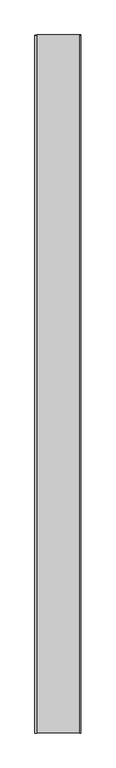
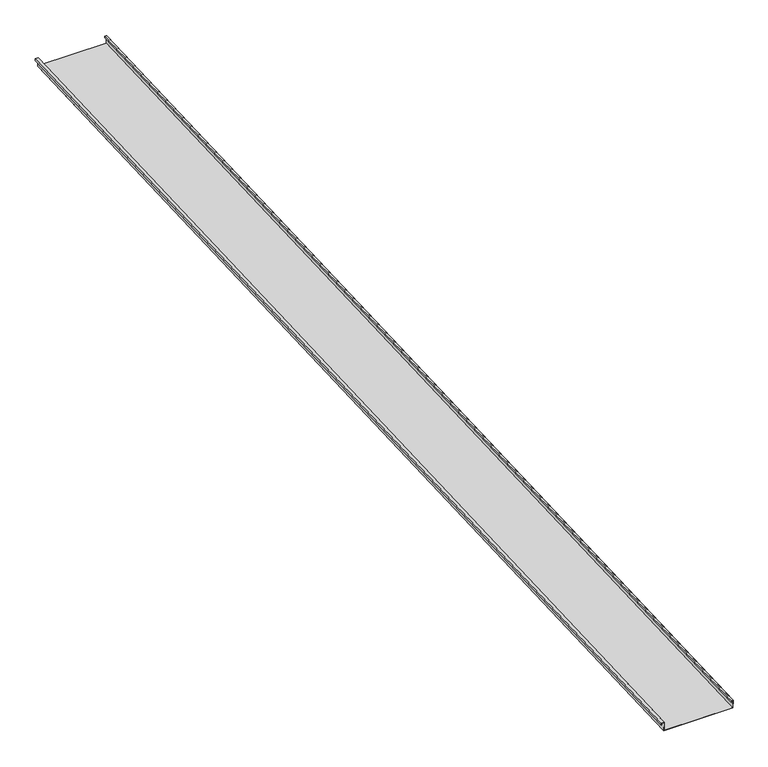
"""IFC4 building model written with IfcOpenShell, lengths in millimetres: proxy geometry, Generic Models 2:Generic Models 2:310765:Generic Models 2:310765 : Generic Models 2:Generic Models 2:310765:124 : Generic Models 2:Generic Models 2:310765:Generic Models 2:310765 : Generic Models 2:Generic Models 2:310765:300385."""

from ifc_helpers import new_model, si_unit, frame, origin, place, context, project, spatial, polyline, outline, extrude, source, transform, mapped, element, save


def generic_models_ac668154(model_context):
    return source(origin(), model_context, "Body", "SweptSolid", [
        extrude(outline(polyline([(1.5875, 0.0), (1.5875, 50.8), (407.9875, 50.8), (407.9875, 1.5875), (396.875, 1.5875), (396.875, 11.1125), (398.4625, 11.1125), (398.4625, 3.175), (406.4, 3.175), (406.4, 49.2125), (3.175, 49.2125), (3.175, -1.5874999), (-14.2875, -1.5874999), (-14.2875, 9.525), (-12.7, 9.525), (-12.7, 0.0), (1.5875, 0.0)])), frame((662984.0429738, -581354.4345603, 3902.6697972), z_axis=(0.0, 0.9991330730923568, 0.041630544712067834), x_axis=(1.0, 0.0, 0.0)), (0.0, 0.0, 1.0), 6400.8),
    ])


if __name__ == "__main__":
    model = new_model("IFC4")
    model_context = context("Model", 3, world=origin())
    ifc_project = project(units=[si_unit("LENGTHUNIT", "METRE", prefix="MILLI")], contexts=[model_context])
    site = spatial("IfcSite", under=ifc_project)
    building = spatial("IfcBuilding", under=site)
    placement = place(None, origin())
    generic_models_shape = generic_models_ac668154(model_context)
    element("IfcBuildingElementProxy", 1, Name="Generic Models 2:Generic Models 2:310765:Generic Models 2:310765 : Generic Models 2:Generic Models 2:310765:124 : Generic Models 2:Generic Models 2:310765:Generic Models 2:310765 : Generic Models 2:Generic Models 2:310765:300385", ObjectType="Generic Models 2:Generic Models 2:310765:Generic Models 2:310765 : Generic Models 2:Generic Models 2:310765:124 : Generic Models 2:Generic Models 2:310765:Generic Models 2:310765 : Generic Models 2:Generic Models 2:310765:300385", at=placement, inside=building, context=model_context, shape_type="MappedRepresentation", body=[
        mapped(generic_models_shape, transform((0.0, 0.0, 0.0), x_axis=(1.0, 0.0, 0.0), y_axis=(0.0, 1.0, 0.0), z_axis=(0.0, 0.0, 1.0))),
    ])
    save(model, "model.ifc")

# Revit data of these elements
# Type "Generic Models 2:Generic Models 2:310765:Generic Models 2:310765 : Generic Models 2:Generic Models 2:310765:124 : Generic Models 2:Generic Models 2:310765:Generic Models 2:310765 : Generic Models 2:Generic Models 2:310765:300385"
#   NameOverride = "Generic Models 2:Generic Models 2:310765:Generic Models 2:310765 : Generic Models 2:Generic Models 2:310765:300385"
#   ObjectTypeOverride = "Generic Models 2:310765 : Generic Models 2:Generic Models 2:310765"
#   Reference = "Generic Models 2"
#   Tag = "300385"
# Element 1 (IfcBuildingElementProxy, "Generic Models 2:Generic Models 2:310765:Generic Models 2:310765 : Generic Models 2:Generic Models 2:310765:124 : Generic Models 2:Generic Models 2:310765:Generic Models 2:310765 : Generic Models 2:Generic Models 2:310765:300385")
#   Materials on its faces: "THERMAL BROKEN ALUMINUM STOREFRONT FOR POLYCARBONATE"
# Materials
#   "THERMAL BROKEN ALUMINUM STOREFRONT FOR POLYCARBONATE": class "Unassigned", colour RGB 244 244 244, transparency 0, Keynote = "M07611300.01", Cost = 0
